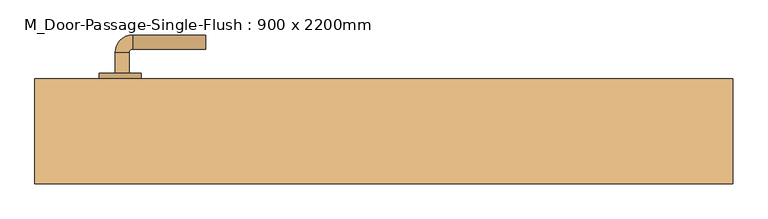
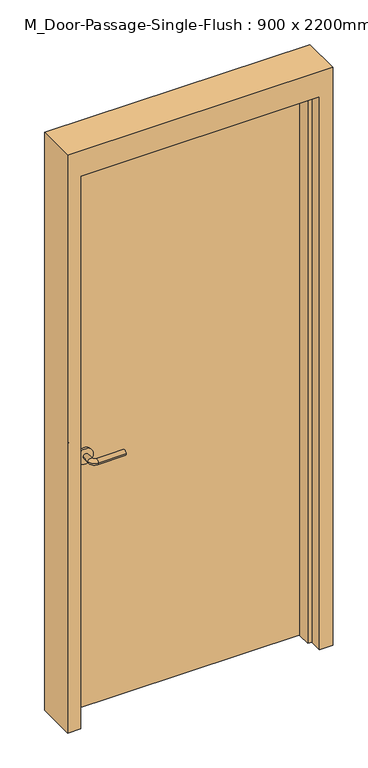
"""IFC4 building model written with IfcOpenShell, lengths in millimetres: door geometry, M_Door-Passage-Single-Flush : 900 x 2200mm."""

from ifc_helpers import new_model, si_unit, point, frame, frame_2d, origin, origin_with_axes, place, context, project, spatial, polyline, circle_curve, ellipse_curve, trimmed, segment, composite_curve, outline, extrude, faceted_brep, source, transform, mapped, element, save
from ifc_brep_helpers import plane_surface, cylinder_surface, revolved_surface, advanced_brep


def m_door_passage_single_flush_900_x_2200mm_ec9e737a(model_context):
    return source(origin(), model_context, "Body", "SolidModel", [
        advanced_brep(
        [(-384.990625, 28.35, 1000.0), (-364.990625, 28.35, 1000.0), (-364.990625, -1.65, 1000.0), (-384.990625, -1.65, 1000.0), (-359.990625, -6.65, 1000.0), (-359.990625, -26.65, 1000.0), (-254.990625, -26.65, 1000.0), (-254.990625, -6.65, 1000.0)],
        [
            (0, 1, circle_curve(frame((-374.990625, 28.35, 1000.0), z_axis=(0.0, 1.0, 0.0), x_axis=(1.0, 0.0, 0.0)), 10.0)),
            (1, 0, circle_curve(frame((-374.990625, 28.35, 1000.0), z_axis=(0.0, 1.0, 0.0), x_axis=(1.0, 0.0, 0.0)), 10.0)),
            (1, 2),
            (2, 3, circle_curve(frame((-374.990625, -1.65, 1000.0), z_axis=(0.0, 1.0, 0.0), x_axis=(1.0, 0.0, 0.0)), 10.0)),
            (3, 0),
            (3, 2, circle_curve(frame((-374.990625, -1.65, 1000.0), z_axis=(0.0, 1.0, 0.0), x_axis=(1.0, 0.0, 0.0)), 10.0)),
            (4, 5, circle_curve(frame((-359.990625, -16.65, 1000.0), z_axis=(-1.0, 0.0, 0.0), x_axis=(0.0, 1.0, 0.0)), 10.0)),
            (5, 3, circle_curve(frame((-359.990625, -1.65, 1000.0), z_axis=(0.0, 0.0, -1.0), x_axis=(-1.0, 0.0, 0.0)), 25.0)),
            (2, 4, circle_curve(frame((-359.990625, -1.65, 1000.0), z_axis=(0.0, 0.0, 1.0), x_axis=(-1.0, 0.0, 0.0)), 5.0)),
            (5, 4, circle_curve(frame((-359.990625, -16.65, 1000.0), z_axis=(-1.0, 0.0, 0.0), x_axis=(0.0, 1.0, 0.0)), 10.0)),
            (6, 7, circle_curve(frame((-254.990625, -16.65, 1000.0), z_axis=(1.0, 0.0, 0.0), x_axis=(0.0, 1.0, 0.0)), 10.0)),
            (7, 6, circle_curve(frame((-254.990625, -16.65, 1000.0), z_axis=(1.0, 0.0, 0.0), x_axis=(0.0, 1.0, 0.0)), 10.0)),
            (4, 7),
            (6, 5),
        ],
        [
            plane_surface(frame((-374.990625, 28.35, 1000.0), z_axis=(0.0, 1.0, 0.0), x_axis=(0.0, 0.0, 1.0))),
            cylinder_surface(frame((-374.990625, 28.35, 1000.0), z_axis=(0.0, 1.0, 0.0), x_axis=(1.0, 0.0, 0.0)), 10.0),
            revolved_surface(trimmed(ellipse_curve(frame((-374.990625, -1.65, 1000.0), z_axis=(0.0, -1.0, 0.0), x_axis=(1.0, 0.0, 0.0)), 10.0, 10.0), [point((-384.990625, -1.65, 1000.0))], [point((-364.990625, -1.65, 1000.0))], True, "CARTESIAN"), (-359.990625, -1.65, 1000.0), (0.0, 0.0, -1.0)),
            revolved_surface(trimmed(ellipse_curve(frame((-374.990625, -1.65, 1000.0), z_axis=(0.0, -1.0, 0.0), x_axis=(1.0, 0.0, 0.0)), 10.0, 10.0), [point((-364.990625, -1.65, 1000.0))], [point((-384.990625, -1.65, 1000.0))], True, "CARTESIAN"), (-359.990625, -1.65, 1000.0), (0.0, 0.0, -1.0)),
            plane_surface(frame((-254.990625, -16.65, 1000.0), z_axis=(1.0, 0.0, 0.0), x_axis=(0.0, 0.0, 1.0))),
            cylinder_surface(frame((-359.990625, -16.65, 1000.0), z_axis=(-1.0, 0.0, 0.0), x_axis=(0.0, 1.0, 0.0)), 10.0),
        ],
        [
            (0, [[1, 2]]),
            (1, [[3, 4, 5, -2]]),
            (1, [[-5, 6, -3, -1]]),
            (2, [[7, 8, -4, 9]]),
            (3, [[10, -9, -6, -8]]),
            (4, [[11, 12]]),
            (5, [[13, -11, 14, -7]]),
            (5, [[-14, -12, -13, -10]]),
        ],
    ),
        extrude(outline(composite_curve([segment(trimmed(circle_curve(frame_2d((1000.0, -377.490625)), 30.0), [point((1000.0, -407.490625))], [point((1000.0, -347.490625))], False, "CARTESIAN"), True, "CONTINUOUS"), segment(trimmed(circle_curve(frame_2d((1000.0, -377.490625)), 30.0), [point((1000.0, -347.490625))], [point((1000.0, -407.490625))], False, "CARTESIAN"), True, "CONTINUOUS")], self_intersect=False)), frame((0.0, 28.35, 0.0), z_axis=(0.0, 1.0, 0.0), x_axis=(0.0, 0.0, 1.0)), (0.0, 0.0, 1.0), 8.0),
        advanced_brep(
        [(-384.990625, 89.35, 1000.0), (-364.990625, 89.35, 1000.0), (-384.990625, 119.35, 1000.0), (-364.990625, 119.35, 1000.0), (-359.990625, 124.35, 1000.0), (-359.990625, 144.35, 1000.0), (-254.990625, 144.35, 1000.0), (-254.990625, 124.35, 1000.0)],
        [
            (0, 1, circle_curve(frame((-374.990625, 89.35, 1000.0), z_axis=(0.0, -1.0, 0.0), x_axis=(1.0, 0.0, 0.0)), 10.0)),
            (1, 0, circle_curve(frame((-374.990625, 89.35, 1000.0), z_axis=(0.0, -1.0, 0.0), x_axis=(1.0, 0.0, 0.0)), 10.0)),
            (0, 2),
            (2, 3, circle_curve(frame((-374.990625, 119.35, 1000.0), z_axis=(0.0, -1.0, 0.0), x_axis=(1.0, 0.0, 0.0)), 10.0)),
            (3, 1),
            (3, 2, circle_curve(frame((-374.990625, 119.35, 1000.0), z_axis=(0.0, -1.0, 0.0), x_axis=(1.0, 0.0, 0.0)), 10.0)),
            (4, 3, circle_curve(frame((-359.990625, 119.35, 1000.0), z_axis=(0.0, 0.0, 1.0), x_axis=(-1.0, 0.0, 0.0)), 5.0)),
            (2, 5, circle_curve(frame((-359.990625, 119.35, 1000.0), z_axis=(0.0, 0.0, -1.0), x_axis=(-1.0, 0.0, 0.0)), 25.0)),
            (5, 4, circle_curve(frame((-359.990625, 134.35, 1000.0), z_axis=(-1.0, 0.0, 0.0), x_axis=(0.0, -1.0, 0.0)), 10.0)),
            (4, 5, circle_curve(frame((-359.990625, 134.35, 1000.0), z_axis=(-1.0, 0.0, 0.0), x_axis=(0.0, -1.0, 0.0)), 10.0)),
            (6, 7, circle_curve(frame((-254.990625, 134.35, 1000.0), z_axis=(1.0, 0.0, 0.0), x_axis=(0.0, -1.0, 0.0)), 10.0)),
            (7, 6, circle_curve(frame((-254.990625, 134.35, 1000.0), z_axis=(1.0, 0.0, 0.0), x_axis=(0.0, -1.0, 0.0)), 10.0)),
            (5, 6),
            (7, 4),
        ],
        [
            plane_surface(frame((-374.990625, 89.35, 1000.0), z_axis=(0.0, -1.0, 0.0), x_axis=(0.0, 0.0, 1.0))),
            cylinder_surface(frame((-374.990625, 89.35, 1000.0), z_axis=(0.0, -1.0, 0.0), x_axis=(1.0, 0.0, 0.0)), 10.0),
            revolved_surface(trimmed(ellipse_curve(frame((-374.990625, 119.35, 1000.0), z_axis=(0.0, -1.0, 0.0), x_axis=(1.0, 0.0, 0.0)), 10.0, 10.0), [point((-384.990625, 119.35, 1000.0))], [point((-364.990625, 119.35, 1000.0))], True, "CARTESIAN"), (-359.990625, 119.35, 1000.0), (0.0, 0.0, -1.0)),
            revolved_surface(trimmed(ellipse_curve(frame((-374.990625, 119.35, 1000.0), z_axis=(0.0, -1.0, 0.0), x_axis=(1.0, 0.0, 0.0)), 10.0, 10.0), [point((-364.990625, 119.35, 1000.0))], [point((-384.990625, 119.35, 1000.0))], True, "CARTESIAN"), (-359.990625, 119.35, 1000.0), (0.0, 0.0, -1.0)),
            plane_surface(frame((-254.990625, 134.35, 1000.0), z_axis=(1.0, 0.0, 0.0), x_axis=(0.0, 0.0, 1.0))),
            cylinder_surface(frame((-359.990625, 134.35, 1000.0), z_axis=(-1.0, 0.0, 0.0), x_axis=(0.0, -1.0, 0.0)), 10.0),
        ],
        [
            (0, [[1, 2]]),
            (1, [[-1, 3, 4, 5]]),
            (1, [[-2, -5, 6, -3]]),
            (2, [[7, -4, 8, 9]]),
            (3, [[-8, -6, -7, 10]]),
            (4, [[11, 12]]),
            (5, [[-9, 13, -12, 14]]),
            (5, [[-10, -14, -11, -13]]),
        ],
    ),
        extrude(outline(composite_curve([segment(trimmed(circle_curve(frame_2d((1000.0, -377.490625)), 30.0), [point((1000.0, -407.490625))], [point((1000.0, -347.490625))], False, "CARTESIAN"), True, "CONTINUOUS"), segment(trimmed(circle_curve(frame_2d((1000.0, -377.490625)), 30.0), [point((1000.0, -347.490625))], [point((1000.0, -407.490625))], False, "CARTESIAN"), True, "CONTINUOUS")], self_intersect=False)), frame((0.0, 81.35, 0.0), z_axis=(0.0, 1.0, 0.0), x_axis=(0.0, 0.0, 1.0)), (0.0, 0.0, 1.0), 8.0),
        extrude(outline(polyline([(450.0, 36.35), (-450.0, 36.35), (-450.0, 81.35), (450.0, 81.35), (450.0, 36.35)])), origin_with_axes(), (0.0, 0.0, 1.0), 2200.0),
        faceted_brep([(450.0, 31.5875, 0.0), (450.0, 81.35, 0.0), (500.0, 81.35, 0.0), (500.0, -68.65, 0.0), (450.0, -68.65, 0.0), (450.0, -19.4375, 0.0), (434.125, -19.4375, 0.0), (434.125, 31.5875, 0.0), (450.0, 31.5875, 2200.0), (450.0, 81.35, 2200.0), (-450.0, 81.35, 2200.0), (-450.0, 81.35, 0.0), (-500.0, 81.35, 0.0), (-500.0, 81.35, 2300.0), (500.0, 81.35, 2300.0), (500.0, -68.65, 2300.0), (-500.0, -68.65, 2300.0), (-500.0, -68.65, 0.0), (-450.0, -68.65, 0.0), (-450.0, -68.65, 2200.0), (450.0, -68.65, 2200.0), (450.0, -19.4375, 2200.0), (-450.0, -19.4375, 2200.0), (-450.0, -19.4375, 0.0), (-434.125, -19.4375, 0.0), (-434.125, -19.4375, 2184.125), (434.125, -19.4375, 2184.125), (434.125, 31.5875, 2184.125), (-434.125, 31.5875, 2184.125), (-434.125, 31.5875, 0.0), (-450.0, 31.5875, 0.0), (-450.0, 31.5875, 2200.0)], [[[0, 1, 2, 3, 4, 5, 6, 7]], [[1, 0, 8, 9]], [[2, 1, 9, 10, 11, 12, 13, 14]], [[3, 2, 14, 15]], [[4, 3, 15, 16, 17, 18, 19, 20]], [[5, 4, 20, 21]], [[6, 5, 21, 22, 23, 24, 25, 26]], [[7, 6, 26, 27]], [[0, 7, 27, 28, 29, 30, 31, 8]], [[9, 8, 31, 10]], [[20, 19, 22, 21]], [[26, 25, 28, 27]], [[12, 11, 30, 29, 24, 23, 18, 17]], [[11, 10, 31, 30]], [[13, 12, 17, 16]], [[19, 18, 23, 22]], [[25, 24, 29, 28]], [[15, 14, 13, 16]]]),
    ])


if __name__ == "__main__":
    model = new_model("IFC4")
    model_context = context("Model", 3, world=origin())
    ifc_project = project(units=[si_unit("LENGTHUNIT", "METRE", prefix="MILLI")], contexts=[model_context])
    site = spatial("IfcSite", under=ifc_project)
    building = spatial("IfcBuilding", under=site)
    placement = place(None, origin())
    m_door_passage_single_flush_900_x_2200mm_shape = m_door_passage_single_flush_900_x_2200mm_ec9e737a(model_context)
    element("IfcDoor", 1, ObjectType="M_Door-Passage-Single-Flush : 900 x 2200mm", at=placement, inside=building, context=model_context, shape_type="MappedRepresentation", body=[
        mapped(m_door_passage_single_flush_900_x_2200mm_shape, transform((0.0, 0.0, 0.0), x_axis=(1.0, 0.0, 0.0), y_axis=(0.0, 1.0, 0.0), z_axis=(0.0, 0.0, 1.0))),
    ])
    save(model, "model.ifc")

# Revit data of these elements
# Type "M_Door-Passage-Single-Flush : 900 x 2200mm"
#   Type Mark = "39"
#   Analytic Construction = "Wooden"
#   Thickness = 45 mm
#   Thermal Resistance (R) = 0.455703 (m²·K)/W
#   Swing Angle [instance default] = 90.00°
#   Strike Height = 1000 mm
#   Rough Width [instance default] = 1000 mm
#   Rough Height [instance default] = 2300 mm
#   MF Opening Height [instance default] = 100 mm
#   MF Opening Width [instance default] = 100 mm
#   Inset Calculate [instance default] = 105 mm
#   Masonry Inset [instance default] = 25 mm
#   Height = 2200 mm
#   Width = 900 mm
#   Heat Transfer Coefficient (U) = 2.19465 W/(m²·K)
#   Masonry Frame Depth = 150 mm
#   Masonry Frame [instance default] = yes
#   Function = 1
#   Dry Wall Frame [instance default] = no
#   Panel Material = Wood - Birch
#   Frame Material = Metal - Paint Finish - Grey
#   Door Handle Material = Aluminum
#   Visual Light Transmittance = 0
#   Solar Heat Gain Coefficient = 0
#   Wall Closure = (empty or 0)
# Element 1 (IfcDoor, "M_Door-Passage-Single-Flush : 900 x 2200mm")
#   Materials on its faces: "Aluminum", "Metal - Paint Finish - Grey", "Wood - Birch"
# Materials
#   "Wood - Birch": class "Wood", colour RGB 173 132 96, transparency 0, Cost = 0
#   "Metal - Paint Finish - Grey": class "Paint", colour RGB 178 178 178, transparency 0, Cost = 0
#   "Aluminum": class "Metal", colour RGB 244 245 246, transparency 0, Description = "Aluminum 6061", Cost = 0
